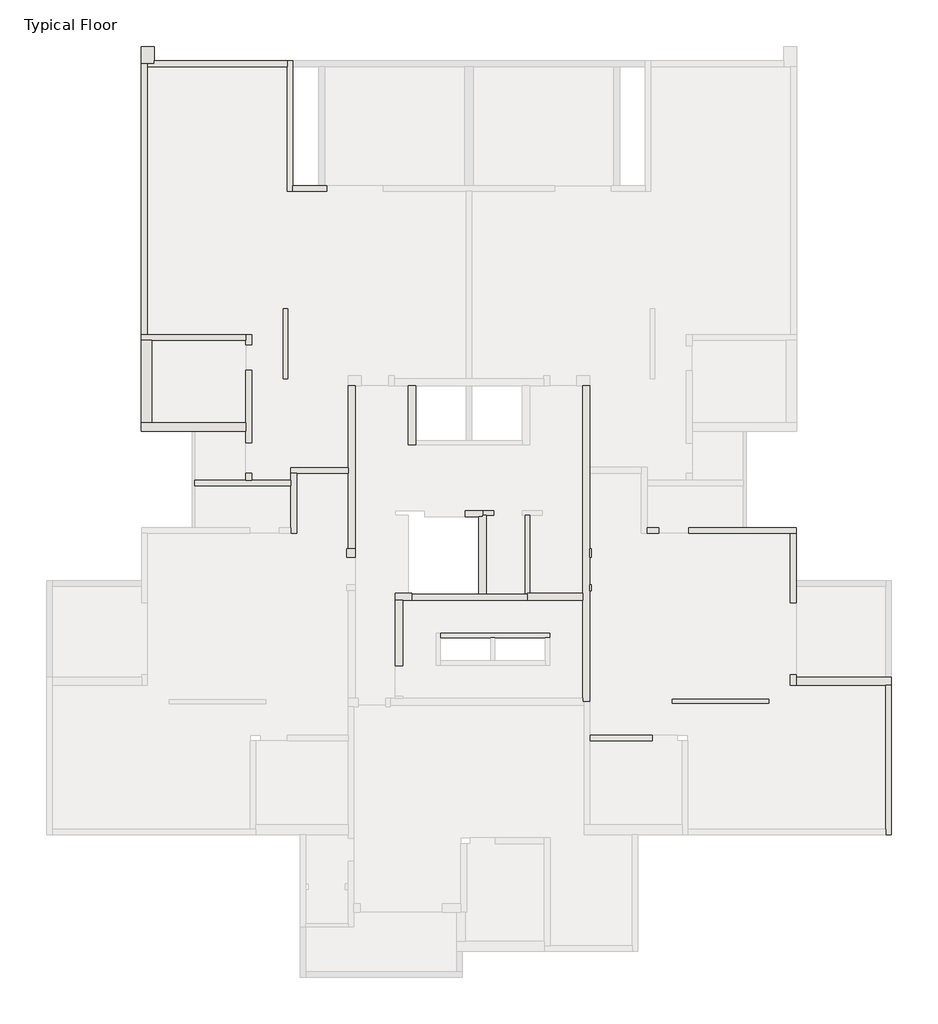
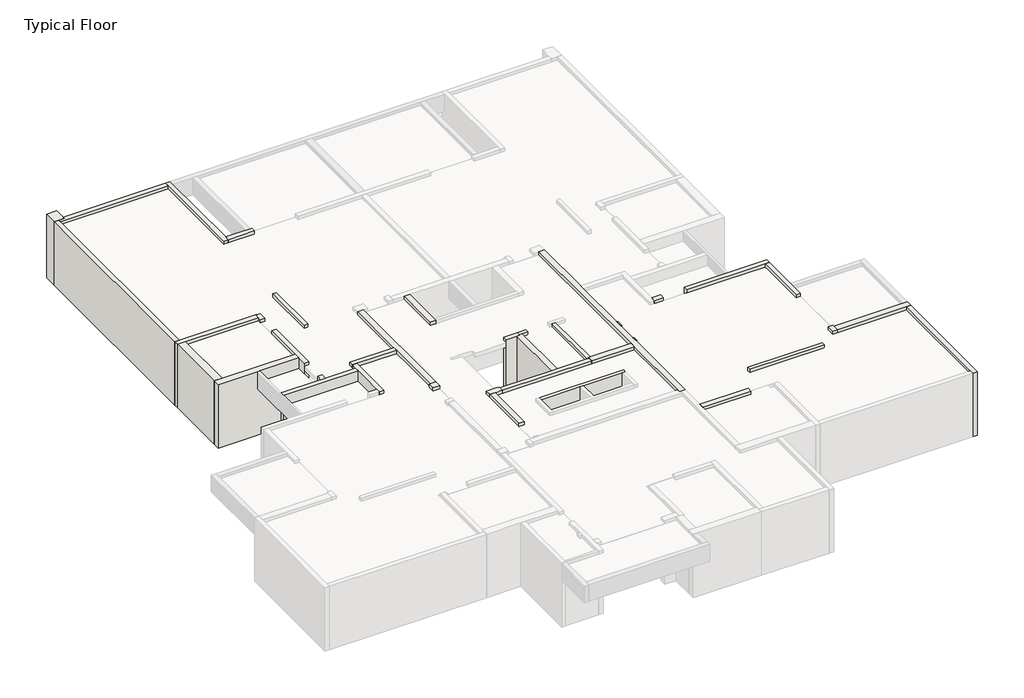
# One storey, part 2 of 4: 38 walls.
# Revit data of these elements (continued)
# Element 36 (IfcWall, "30") (continued)
#   SOFiSTiK_AMG_Comments = "Too Short /"
#   built-in parameter 1001111 = -300 cm
#   Top Offset = 0 cm
#   Base Offset = -300 cm
#   wall height = 300 cm
#   SOFiSTiK_AMG_Scheduled = yes
#   SOFiSTiK_AMG_Adjusted = yes
#   Phase Created = New Construction
#   Base Constraint = Typical Floor
#   Top Constraint = Typical Floor
#   Materials on its faces: "Concrete, Cast-in-Place - B30"
# Element 37 (IfcWall, "35")
#   Comments = ""
#   Mark = "W69"
#   SOFiSTiK_AMG_Comments = ""
#   built-in parameter 1001111 = -300 cm
#   Top Offset = 0 cm
#   Base Offset = -300 cm
#   wall height = 300 cm
#   SOFiSTiK_AMG_Scheduled = yes
#   SOFiSTiK_AMG_Adjusted = yes
#   Phase Created = New Construction
#   Base Constraint = Typical Floor
#   Top Constraint = Typical Floor
#   Materials on its faces: "Concrete, Cast-in-Place - B30"
# Element 38 (IfcWall, "45")
#   Comments = ""
#   Mark = "W75"
#   SOFiSTiK_AMG_Comments = ""
#   built-in parameter 1001111 = -300 cm
#   Top Offset = 0 cm
#   Base Offset = -300 cm
#   wall height = 300 cm
#   SOFiSTiK_AMG_Scheduled = yes
#   SOFiSTiK_AMG_Adjusted = yes
#   Phase Created = New Construction
#   Base Constraint = Typical Floor
#   Top Constraint = Typical Floor
#   Materials on its faces: "Concrete, Cast-in-Place - B30"
# Materials
#   "Concrete, Cast-in-Place - B30": class "Concrete", colour RGB 192 192 192, transparency 0, Keynote = "01000", Description = "Cast-in-place concrete", Cost = 0
